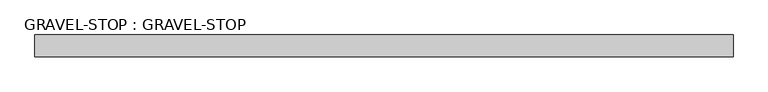
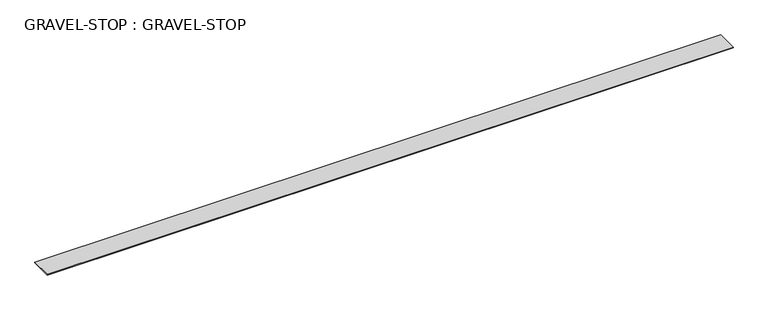
"""IFC4 building model written with IfcOpenShell, lengths in millimetres: proxy geometry, GRAVEL-STOP : GRAVEL-STOP."""

from ifc_helpers import new_model, si_unit, frame, origin, place, context, project, spatial, polyline, outline, extrude, source, transform, mapped, element, save


def gravel_stop_gravel_stop_6292a2d3(model_context):
    return source(origin(), model_context, "Body", "SweptSolid", [
        extrude(outline(polyline([(12382.7678845, -5509.5258868), (12382.7678845, -5447.1977788), (14383.0178845, -5447.1977788), (14383.0178845, -5509.5258868), (12382.7678845, -5509.5258868)])), frame((0.0, 0.0, 40237.274455), z_axis=(0.0, 0.0, 1.0), x_axis=(1.0, 0.0, 0.0)), (0.0, 0.0, 1.0), 2.3397091),
    ])


if __name__ == "__main__":
    model = new_model("IFC4")
    model_context = context("Model", 3, world=origin())
    ifc_project = project(units=[si_unit("LENGTHUNIT", "METRE", prefix="MILLI")], contexts=[model_context])
    site = spatial("IfcSite", under=ifc_project)
    building = spatial("IfcBuilding", under=site)
    placement = place(None, origin())
    gravel_stop_gravel_stop_shape = gravel_stop_gravel_stop_6292a2d3(model_context)
    element("IfcBuildingElementProxy", 1, Name="GRAVEL-STOP : GRAVEL-STOP", ObjectType="GRAVEL-STOP : GRAVEL-STOP", at=placement, inside=building, context=model_context, shape_type="MappedRepresentation", body=[
        mapped(gravel_stop_gravel_stop_shape, transform((0.0, 0.0, 0.0), x_axis=(1.0, 0.0, 0.0), y_axis=(0.0, 1.0, 0.0), z_axis=(0.0, 0.0, 1.0))),
    ])
    save(model, "model.ifc")

# Revit data of these elements
# Type "GRAVEL-STOP : GRAVEL-STOP"
#   NameOverride = "GRAVEL-STOP"
# Element 1 (IfcBuildingElementProxy, "GRAVEL-STOP : GRAVEL-STOP")
#   Materials on its faces: "METAL FLASHING"
# Materials
#   "METAL FLASHING": class "Unassigned", colour RGB 128 128 128, transparency 0
